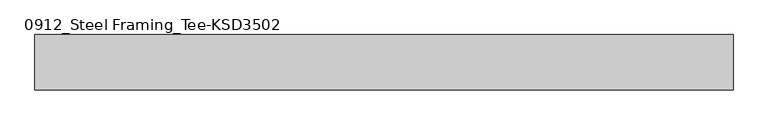
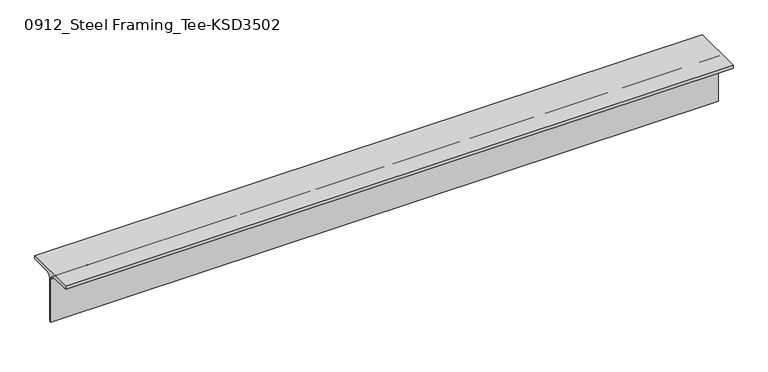
"""IFC4 building model written with IfcOpenShell, lengths in millimetres: member geometry, 0912_Steel Framing_Tee-KSD3502 : H_SB_ASB_CT-150x150x6.5x9."""

from ifc_helpers import new_model, si_unit, point, frame, frame_2d, origin, place, context, project, spatial, polyline, circle_curve, trimmed, segment, composite_curve, outline, extrude, source, transform, mapped, element, save


def member_0912_steel_framing_tee_ksd3502_dc475893(model_context):
    return source(origin(), model_context, "Body", "SweptSolid", [
        extrude(outline(composite_curve([segment(polyline([(-75.0, 75.0), (75.0, 75.0), (75.0, 66.0), (16.25, 66.0)]), True, "CONTINUOUS"), segment(trimmed(circle_curve(frame_2d((16.25, 53.0)), 13.0), [point((16.25, 66.0))], [point((3.25, 53.0))], True, "CARTESIAN"), True, "CONTINUOUS"), segment(polyline([(3.25, 53.0), (3.25, -75.0), (-3.25, -75.0), (-3.25, 53.0)]), True, "CONTINUOUS"), segment(trimmed(circle_curve(frame_2d((-16.25, 53.0)), 13.0), [point((-3.25, 53.0))], [point((-16.25, 66.0))], True, "CARTESIAN"), True, "CONTINUOUS"), segment(polyline([(-16.25, 66.0), (-75.0, 66.0), (-75.0, 75.0)]), True, "CONTINUOUS")], self_intersect=False)), frame((-983.95, 0.0, 0.0), z_axis=(1.0, 0.0, 0.0), x_axis=(0.0, 1.0, 0.0)), (0.0, 0.0, 1.0), 1884.0),
    ])


if __name__ == "__main__":
    model = new_model("IFC4")
    model_context = context("Model", 3, world=origin())
    ifc_project = project(units=[si_unit("LENGTHUNIT", "METRE", prefix="MILLI")], contexts=[model_context])
    site = spatial("IfcSite", under=ifc_project)
    building = spatial("IfcBuilding", under=site)
    placement = place(None, origin())
    member_0912_steel_framing_tee_ksd3502_shape = member_0912_steel_framing_tee_ksd3502_dc475893(model_context)
    element("IfcMember", 1, ObjectType="0912_Steel Framing_Tee-KSD3502 : H_SB_ASB_CT-150x150x6.5x9", at=placement, inside=building, context=model_context, shape_type="MappedRepresentation", body=[
        mapped(member_0912_steel_framing_tee_ksd3502_shape, transform((0.0, 0.0, 0.0), x_axis=(1.0, 0.0, 0.0), y_axis=(0.0, 1.0, 0.0), z_axis=(0.0, 0.0, 1.0))),
    ])
    save(model, "model.ifc")

# Revit data of these elements
# Type "0912_Steel Framing_Tee-KSD3502 : H_SB_ASB_CT-150x150x6.5x9"
#   H_WM Code_1 = "S01AA003-00001 | Main Steel Structure Fabrication Work | Shelter/Building | Light Steel - Standard (30KG/M>Weight) | Material: (   )"
#   H_WM Code_2 = "S03AA029-00001 | Main Steel Structure Erection Work | Shelter/Building | Light Steel (30KG/M>Weight) | Material: (   )"
#   H_WM Code_3 = "S01AA010-00001 | Main Steel Structure Fabrication Work | Shelter/Building | Steel Painting/Coating | for Non-Fireproofed Steel Surface, Surface Preparation, Primer, Second & Final Coat | Material: (   )"
#   H_Q'ty Cal Type Tag = "SB-Q2"
#   Width = 15.0 cm
#   Web Thickness = 0.65 cm
#   Web Fillet = 1.3 cm
#   Section Area = 23.39 cm²
#   Perimeter = 0.60 m²/m
#   Nominal Weight = 18.40 kgf/m
#   Height = 15.0 cm
#   Flange Thickness = 0.9 cm
#   Centroid Vertical = 7.5 cm
#   Centroid Horizontal = 7.5 cm
#   Length [instance default] = 1.5000 m
#   Structural Material [instance default] = Steel, 45-345
#   Warping Constant = (empty or 0)
#   Torsional Moment of Inertia = 0
#   Section Name Key = ""
#   Plastic Modulus weak axis = 0
#   Plastic Modulus strong axis = 0
#   Moment of Inertia weak axis = 0
#   Moment of Inertia strong axis = 0
#   Elastic Modulus weak axis = 0
#   Elastic Modulus strong axis = 0
#   Bolt Spacing = 0
#   Assembly Code = ""
# Element 1 (IfcMember, "0912_Steel Framing_Tee-KSD3502 : H_SB_ASB_CT-150x150x6.5x9")
#   Structural Material = none
# Materials
#   "Steel, 45-345": class "Metal", colour RGB 189 187 185, transparency 0, Description = "Steel 345 MPa", Cost = 0
